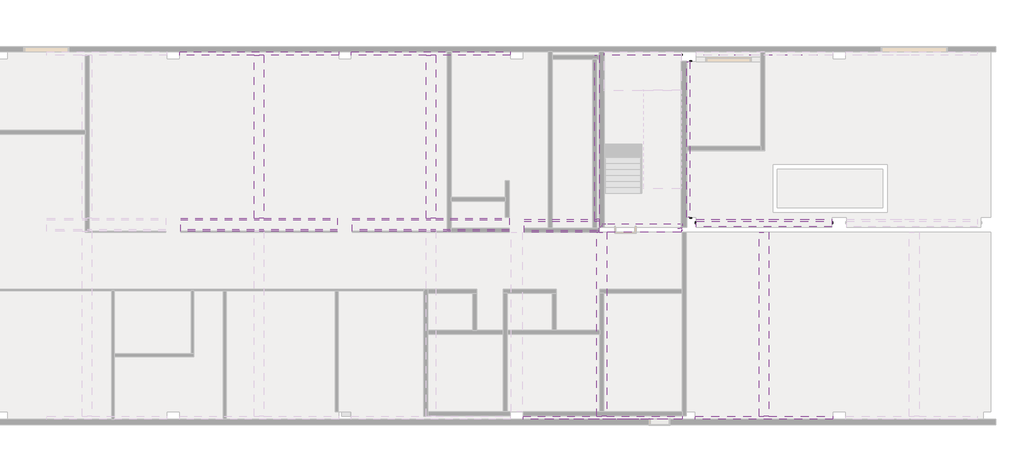
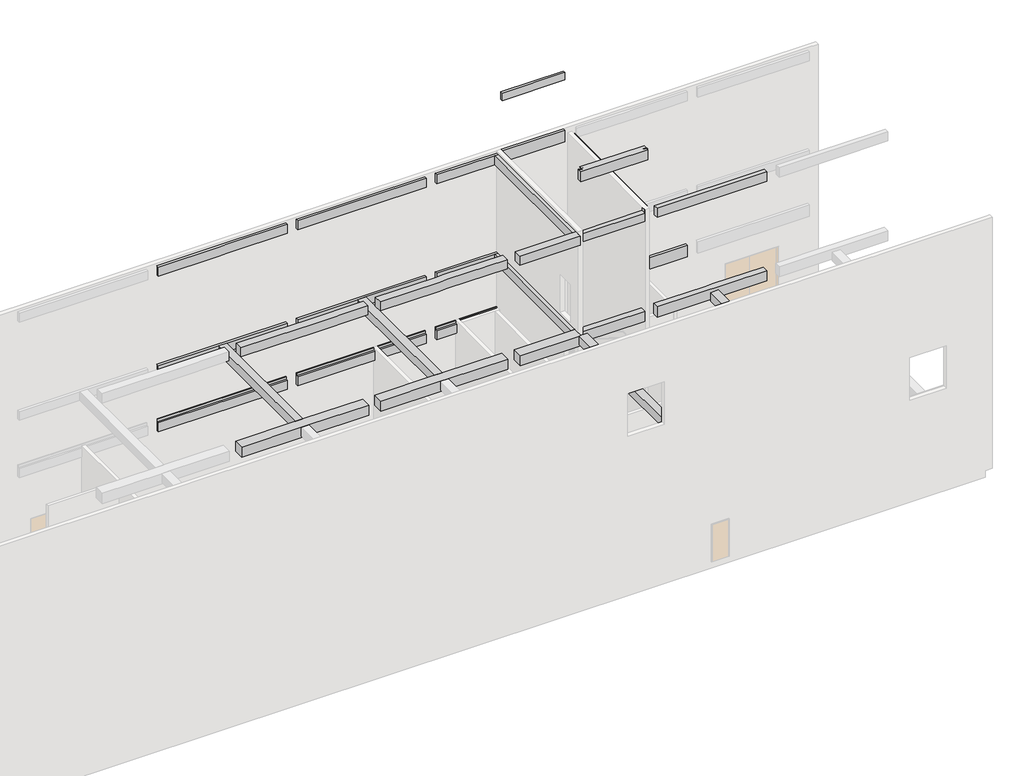
# One storey, part 4 of 5: 55 beams.
# Revit data of these elements (continued)
# Type "RC Beam_Rectangular : H_SB_AR_S16_UG_B500xH700_1G3" (continued)
#   H_WM Code_3 = "A03AF036-00001 |  | M2 | Concrete Work | Superstructure Work | Form Work (1 time in use) | Flat Form | Dressed Lumber, Plywood or Steel Form(Wood Planks are not Allowed) incl. Chamfer |  |  |  | A03AF036-00001 Concrete Work Superstructure Work Form Work (1 time in use) Flat Form     Dressed Lumber, Plywood or Steel Form(Wood Planks are not Allowed) incl. Chamfer   |"
#   중앙부 하부근 = ""
#   중앙부 상부근 = ""
#   중앙부 보조근 = ""
#   중앙부 늑근 = ""
#   외단부 하부근 = ""
#   외단부 상부근 = ""
#   외단부 보조근 = ""
#   외단부 늑근 = ""
#   부호 = "TG2"
#   내단부 하부근 = ""
#   내단부 상부근 = ""
#   내단부 보조근 = ""
#   내단부 늑근 = ""
#   ALL 하부근 = "3-D20"
#   ALL 상부근 = "4-D20"
#   ALL 보조근 = ""
#   ALL 늑근 = "2-D10 @120"
#   H_Rebar ratio = 0.14
#   Width = 500 mm
#   Height = 700 mm
#   Length [instance default] = 1524 mm
#   b = 500 mm
#   h = 700 mm
#   hec_material3 [instance default] = none
#   hec_material2 [instance default] = none
#   hec_material1 [instance default] = none
#   Structural Material [instance default] = none
#   Assembly Code = ""
# Type "RC Beam_Rectangular : H_SB_AR_S16_UG_B600xH800_1G2"
#   Type Comments = "CV-UG"
#   Type Mark = "1G2"
#   H_Q'ty Cal Type Tag = "SB-Q1"
#   H_WM Code_1 = "A03AF032-00022 |  | M3 | Concrete Work | Superstructure Work | Structural Concrete | Cement Type-1 | 25MPa ≤ F'c (Cylinder Strength) < 30MPa |  |  |  |  | A03AF032-00022 Concrete Work Superstructure Work Structural Concrete  Cement Type-1 25MPa ≤ F'c (Cylinder Strength) < 30MPa      |  F'c (Cylinder Strength) = 24MPa"
#   H_WM Code_2 = "A03AD037-00002 |  | TON | Concrete Work | Substructure Work | Rebar Work | Deformed Bar (Non-Coat.) | 400MPa<Fy≤470MPa |  |  |  |  | A03AD037-00002 Concrete Work Substructure Work Rebar Work Deformed Bar (Non-Coat.)  400MPa<Fy≤470MPa      | ASTM A615 GRADE 60 (Fy=420MPa)"
#   H_WM Code_3 = "A03AF036-00001 |  | M2 | Concrete Work | Superstructure Work | Form Work (1 time in use) | Flat Form | Dressed Lumber, Plywood or Steel Form(Wood Planks are not Allowed) incl. Chamfer |  |  |  | A03AF036-00001 Concrete Work Superstructure Work Form Work (1 time in use) Flat Form     Dressed Lumber, Plywood or Steel Form(Wood Planks are not Allowed) incl. Chamfer   |"
#   중앙부 하부근 = ""
#   중앙부 상부근 = ""
#   중앙부 보조근 = ""
#   중앙부 늑근 = ""
#   외단부 하부근 = ""
#   외단부 상부근 = ""
#   외단부 보조근 = ""
#   외단부 늑근 = ""
#   부호 = "TG2"
#   내단부 하부근 = ""
#   내단부 상부근 = ""
#   내단부 보조근 = ""
#   내단부 늑근 = ""
#   ALL 하부근 = "3-D20"
#   ALL 상부근 = "4-D20"
#   ALL 보조근 = ""
#   ALL 늑근 = "2-D10 @120"
#   H_Rebar ratio = 0.14
#   Width = 600 mm
#   Height = 800 mm
#   Length [instance default] = 1524 mm
#   b = 600 mm
#   h = 800 mm
#   hec_material3 [instance default] = none
#   hec_material2 [instance default] = none
#   hec_material1 [instance default] = none
#   Structural Material [instance default] = none
#   Assembly Code = ""
# Type "RC Beam_Rectangular : H_SB_AR_S16_UG_B450xH700_1B1"
#   Type Comments = "CV-UG"
#   Type Mark = "1B1"
#   H_Q'ty Cal Type Tag = "SB-Q1"
#   H_WM Code_1 = "A03AF032-00022 |  | M3 | Concrete Work | Superstructure Work | Structural Concrete | Cement Type-1 | 25MPa ≤ F'c (Cylinder Strength) < 30MPa |  |  |  |  | A03AF032-00022 Concrete Work Superstructure Work Structural Concrete  Cement Type-1 25MPa ≤ F'c (Cylinder Strength) < 30MPa      |  F'c (Cylinder Strength) = 24MPa"
#   H_WM Code_2 = "A03AD037-00002 |  | TON | Concrete Work | Substructure Work | Rebar Work | Deformed Bar (Non-Coat.) | 400MPa<Fy≤470MPa |  |  |  |  | A03AD037-00002 Concrete Work Substructure Work Rebar Work Deformed Bar (Non-Coat.)  400MPa<Fy≤470MPa      | ASTM A615 GRADE 60 (Fy=420MPa)"
#   H_WM Code_3 = "A03AF036-00001 |  | M2 | Concrete Work | Superstructure Work | Form Work (1 time in use) | Flat Form | Dressed Lumber, Plywood or Steel Form(Wood Planks are not Allowed) incl. Chamfer |  |  |  | A03AF036-00001 Concrete Work Superstructure Work Form Work (1 time in use) Flat Form     Dressed Lumber, Plywood or Steel Form(Wood Planks are not Allowed) incl. Chamfer   |"
#   중앙부 하부근 = ""
#   중앙부 상부근 = ""
#   중앙부 보조근 = ""
#   중앙부 늑근 = ""
#   외단부 하부근 = ""
#   외단부 상부근 = ""
#   외단부 보조근 = ""
#   외단부 늑근 = ""
#   부호 = "TG2"
#   내단부 하부근 = ""
#   내단부 상부근 = ""
#   내단부 보조근 = ""
#   내단부 늑근 = ""
#   ALL 하부근 = "3-D20"
#   ALL 상부근 = "4-D20"
#   ALL 보조근 = ""
#   ALL 늑근 = "2-D10 @120"
#   H_Rebar ratio = 0.14
#   Width = 450 mm
#   Height = 700 mm
#   Length [instance default] = 1524 mm
#   b = 450 mm
#   h = 700 mm
#   hec_material3 [instance default] = none
#   hec_material2 [instance default] = none
#   hec_material1 [instance default] = none
#   Structural Material [instance default] = none
#   Assembly Code = ""
# Type "RC Beam_Rectangular : H_SB_AR_S16_AG_B400xH700_3WG1"
#   Type Comments = "CV-AG"
#   Type Mark = "3WG1"
#   H_Q'ty Cal Type Tag = "SB-Q1"
#   H_WM Code_1 = "A03AF032-00022 |  | M3 | Concrete Work | Superstructure Work | Structural Concrete | Cement Type-1 | 25MPa ≤ F'c (Cylinder Strength) < 30MPa |  |  |  |  | A03AF032-00022 Concrete Work Superstructure Work Structural Concrete  Cement Type-1 25MPa ≤ F'c (Cylinder Strength) < 30MPa      |  F'c (Cylinder Strength) = 24MPa"
#   H_WM Code_2 = "A03AD037-00002 |  | TON | Concrete Work | Substructure Work | Rebar Work | Deformed Bar (Non-Coat.) | 400MPa<Fy≤470MPa |  |  |  |  | A03AD037-00002 Concrete Work Substructure Work Rebar Work Deformed Bar (Non-Coat.)  400MPa<Fy≤470MPa      | ASTM A615 GRADE 60 (Fy=420MPa)"
#   H_WM Code_3 = "A03AF036-00001 |  | M2 | Concrete Work | Superstructure Work | Form Work (1 time in use) | Flat Form | Dressed Lumber, Plywood or Steel Form(Wood Planks are not Allowed) incl. Chamfer |  |  |  | A03AF036-00001 Concrete Work Superstructure Work Form Work (1 time in use) Flat Form     Dressed Lumber, Plywood or Steel Form(Wood Planks are not Allowed) incl. Chamfer   |"
#   중앙부 하부근 = ""
#   중앙부 상부근 = ""
#   중앙부 보조근 = ""
#   중앙부 늑근 = ""
#   외단부 하부근 = ""
#   외단부 상부근 = ""
#   외단부 보조근 = ""
#   외단부 늑근 = ""
#   부호 = "TG2"
#   내단부 하부근 = ""
#   내단부 상부근 = ""
#   내단부 보조근 = ""
#   내단부 늑근 = ""
#   ALL 하부근 = "3-D20"
#   ALL 상부근 = "4-D20"
#   ALL 보조근 = ""
#   ALL 늑근 = "2-D10 @120"
#   H_Rebar ratio = 0.14
#   Width = 400 mm
#   Height = 700 mm
#   Length [instance default] = 1524 mm
#   b = 400 mm
#   h = 700 mm
#   hec_material3 [instance default] = none
#   hec_material2 [instance default] = none
#   hec_material1 [instance default] = none
#   Structural Material [instance default] = none
#   Assembly Code = ""
# Type "RC Beam_Rectangular : H_SB_AR_S16_AG_B600xH800_3G2"
#   Type Comments = "AG"
#   Type Mark = "3G2"
#   H_Q'ty Cal Type Tag = "SB-Q1"
#   H_WM Code_1 = "A03AF032-00022 |  | M3 | Concrete Work | Superstructure Work | Structural Concrete | Cement Type-1 | 25MPa ≤ F'c (Cylinder Strength) < 30MPa |  |  |  |  | A03AF032-00022 Concrete Work Superstructure Work Structural Concrete  Cement Type-1 25MPa ≤ F'c (Cylinder Strength) < 30MPa      |  F'c (Cylinder Strength) = 24MPa"
#   H_WM Code_2 = "A03AD037-00002 |  | TON | Concrete Work | Substructure Work | Rebar Work | Deformed Bar (Non-Coat.) | 400MPa<Fy≤470MPa |  |  |  |  | A03AD037-00002 Concrete Work Substructure Work Rebar Work Deformed Bar (Non-Coat.)  400MPa<Fy≤470MPa      | ASTM A615 GRADE 60 (Fy=420MPa)"
#   H_WM Code_3 = "A03AF036-00001 |  | M2 | Concrete Work | Superstructure Work | Form Work (1 time in use) | Flat Form | Dressed Lumber, Plywood or Steel Form(Wood Planks are not Allowed) incl. Chamfer |  |  |  | A03AF036-00001 Concrete Work Superstructure Work Form Work (1 time in use) Flat Form     Dressed Lumber, Plywood or Steel Form(Wood Planks are not Allowed) incl. Chamfer   |"
#   중앙부 하부근 = ""
#   중앙부 상부근 = ""
#   중앙부 보조근 = ""
#   중앙부 늑근 = ""
#   외단부 하부근 = ""
#   외단부 상부근 = ""
#   외단부 보조근 = ""
#   외단부 늑근 = ""
#   부호 = "TG2"
#   내단부 하부근 = ""
#   내단부 상부근 = ""
#   내단부 보조근 = ""
#   내단부 늑근 = ""
#   ALL 하부근 = "3-D20"
#   ALL 상부근 = "4-D20"
#   ALL 보조근 = ""
#   ALL 늑근 = "2-D10 @120"
#   Width = 600 mm
#   Height = 800 mm
#   Length [instance default] = 1524 mm
#   b = 600 mm
#   h = 800 mm
#   hec_material3 [instance default] = none
#   hec_material2 [instance default] = none
#   hec_material1 [instance default] = none
#   Structural Material [instance default] = none
#   Assembly Code = ""
# Type "RC Beam_Rectangular : H_SB_AR_S16_AG_B600xH800_3WG2"
#   Type Comments = "AG"
#   Type Mark = "3WG2"
#   H_Q'ty Cal Type Tag = "SB-Q1"
#   H_WM Code_1 = "A03AF032-00022 |  | M3 | Concrete Work | Superstructure Work | Structural Concrete | Cement Type-1 | 25MPa ≤ F'c (Cylinder Strength) < 30MPa |  |  |  |  | A03AF032-00022 Concrete Work Superstructure Work Structural Concrete  Cement Type-1 25MPa ≤ F'c (Cylinder Strength) < 30MPa      |  F'c (Cylinder Strength) = 24MPa"
#   H_WM Code_2 = "A03AD037-00002 |  | TON | Concrete Work | Substructure Work | Rebar Work | Deformed Bar (Non-Coat.) | 400MPa<Fy≤470MPa |  |  |  |  | A03AD037-00002 Concrete Work Substructure Work Rebar Work Deformed Bar (Non-Coat.)  400MPa<Fy≤470MPa      | ASTM A615 GRADE 60 (Fy=420MPa)"
#   H_WM Code_3 = "A03AF036-00001 |  | M2 | Concrete Work | Superstructure Work | Form Work (1 time in use) | Flat Form | Dressed Lumber, Plywood or Steel Form(Wood Planks are not Allowed) incl. Chamfer |  |  |  | A03AF036-00001 Concrete Work Superstructure Work Form Work (1 time in use) Flat Form     Dressed Lumber, Plywood or Steel Form(Wood Planks are not Allowed) incl. Chamfer   |"
#   중앙부 하부근 = ""
#   중앙부 상부근 = ""
#   중앙부 보조근 = ""
#   중앙부 늑근 = ""
#   외단부 하부근 = ""
#   외단부 상부근 = ""
#   외단부 보조근 = ""
#   외단부 늑근 = ""
#   부호 = "TG2"
#   내단부 하부근 = ""
#   내단부 상부근 = ""
#   내단부 보조근 = ""
#   내단부 늑근 = ""
#   ALL 하부근 = "3-D20"
#   ALL 상부근 = "4-D20"
#   ALL 보조근 = ""
#   ALL 늑근 = "2-D10 @120"
#   Width = 600 mm
#   Height = 800 mm
#   Length [instance default] = 1524 mm
#   b = 600 mm
#   h = 800 mm
#   hec_material3 [instance default] = none
#   hec_material2 [instance default] = none
#   hec_material1 [instance default] = none
#   Structural Material [instance default] = none
#   Assembly Code = ""
# Type "RC Beam_Rectangular : H_SB_AR_S16_AG_B400xH700_3WG3"
#   Type Comments = "AG"
#   Type Mark = "3WG3"
#   H_Q'ty Cal Type Tag = "SB-Q1"
#   H_WM Code_1 = "A03AF032-00022 |  | M3 | Concrete Work | Superstructure Work | Structural Concrete | Cement Type-1 | 25MPa ≤ F'c (Cylinder Strength) < 30MPa |  |  |  |  | A03AF032-00022 Concrete Work Superstructure Work Structural Concrete  Cement Type-1 25MPa ≤ F'c (Cylinder Strength) < 30MPa      |  F'c (Cylinder Strength) = 24MPa"
#   H_WM Code_2 = "A03AD037-00002 |  | TON | Concrete Work | Substructure Work | Rebar Work | Deformed Bar (Non-Coat.) | 400MPa<Fy≤470MPa |  |  |  |  | A03AD037-00002 Concrete Work Substructure Work Rebar Work Deformed Bar (Non-Coat.)  400MPa<Fy≤470MPa      | ASTM A615 GRADE 60 (Fy=420MPa)"
#   H_WM Code_3 = "A03AF036-00001 |  | M2 | Concrete Work | Superstructure Work | Form Work (1 time in use) | Flat Form | Dressed Lumber, Plywood or Steel Form(Wood Planks are not Allowed) incl. Chamfer |  |  |  | A03AF036-00001 Concrete Work Superstructure Work Form Work (1 time in use) Flat Form     Dressed Lumber, Plywood or Steel Form(Wood Planks are not Allowed) incl. Chamfer   |"
#   중앙부 하부근 = ""
#   중앙부 상부근 = ""
#   중앙부 보조근 = ""
#   중앙부 늑근 = ""
#   외단부 하부근 = ""
#   외단부 상부근 = ""
#   외단부 보조근 = ""
#   외단부 늑근 = ""
#   부호 = "TG2"
#   내단부 하부근 = ""
#   내단부 상부근 = ""
#   내단부 보조근 = ""
#   내단부 늑근 = ""
#   ALL 하부근 = "3-D20"
#   ALL 상부근 = "4-D20"
#   ALL 보조근 = ""
#   ALL 늑근 = "2-D10 @120"
#   Width = 400 mm
#   Height = 700 mm
#   Length [instance default] = 1524 mm
#   b = 400 mm
#   h = 700 mm
#   hec_material3 [instance default] = none
#   hec_material2 [instance default] = none
#   hec_material1 [instance default] = none
#   Structural Material [instance default] = none
#   Assembly Code = ""
# Type "RC Beam_Rectangular : H_SB_AR_S16_AG_B450xH700_2WB1"
#   Type Comments = "AG"
#   Type Mark = "2WB1"
#   H_Q'ty Cal Type Tag = "SB-Q1"
#   H_WM Code_1 = "A03AF032-00022 |  | M3 | Concrete Work | Superstructure Work | Structural Concrete | Cement Type-1 | 25MPa ≤ F'c (Cylinder Strength) < 30MPa |  |  |  |  | A03AF032-00022 Concrete Work Superstructure Work Structural Concrete  Cement Type-1 25MPa ≤ F'c (Cylinder Strength) < 30MPa      |  F'c (Cylinder Strength) = 24MPa"
#   H_WM Code_2 = "A03AD037-00002 |  | TON | Concrete Work | Substructure Work | Rebar Work | Deformed Bar (Non-Coat.) | 400MPa<Fy≤470MPa |  |  |  |  | A03AD037-00002 Concrete Work Substructure Work Rebar Work Deformed Bar (Non-Coat.)  400MPa<Fy≤470MPa      | ASTM A615 GRADE 60 (Fy=420MPa)"
#   H_WM Code_3 = "A03AF036-00001 |  | M2 | Concrete Work | Superstructure Work | Form Work (1 time in use) | Flat Form | Dressed Lumber, Plywood or Steel Form(Wood Planks are not Allowed) incl. Chamfer |  |  |  | A03AF036-00001 Concrete Work Superstructure Work Form Work (1 time in use) Flat Form     Dressed Lumber, Plywood or Steel Form(Wood Planks are not Allowed) incl. Chamfer   |"
#   중앙부 하부근 = ""
#   중앙부 상부근 = ""
#   중앙부 보조근 = ""
#   중앙부 늑근 = ""
#   외단부 하부근 = ""
#   외단부 상부근 = ""
#   외단부 보조근 = ""
#   외단부 늑근 = ""
#   부호 = "TG2"
#   내단부 하부근 = ""
#   내단부 상부근 = ""
#   내단부 보조근 = ""
#   내단부 늑근 = ""
#   ALL 하부근 = "3-D20"
#   ALL 상부근 = "4-D20"
#   ALL 보조근 = ""
#   ALL 늑근 = "2-D10 @120"
#   Width = 450 mm
#   Height = 700 mm
#   Length [instance default] = 1524 mm
#   b = 450 mm
#   h = 700 mm
#   hec_material3 [instance default] = none
#   hec_material2 [instance default] = none
#   hec_material1 [instance default] = none
#   Structural Material [instance default] = none
#   Assembly Code = ""
# Type "RC Beam_Rectangular : H_SB_AR_S16_AG_B450xH700_3B1"
#   Type Comments = "AG"
#   Type Mark = "3B1"
#   H_Q'ty Cal Type Tag = "SB-Q1"
#   H_WM Code_1 = "A03AF032-00022 |  | M3 | Concrete Work | Superstructure Work | Structural Concrete | Cement Type-1 | 25MPa ≤ F'c (Cylinder Strength) < 30MPa |  |  |  |  | A03AF032-00022 Concrete Work Superstructure Work Structural Concrete  Cement Type-1 25MPa ≤ F'c (Cylinder Strength) < 30MPa      |  F'c (Cylinder Strength) = 24MPa"
#   H_WM Code_2 = "A03AD037-00002 |  | TON | Concrete Work | Substructure Work | Rebar Work | Deformed Bar (Non-Coat.) | 400MPa<Fy≤470MPa |  |  |  |  | A03AD037-00002 Concrete Work Substructure Work Rebar Work Deformed Bar (Non-Coat.)  400MPa<Fy≤470MPa      | ASTM A615 GRADE 60 (Fy=420MPa)"
#   H_WM Code_3 = "A03AF036-00001 |  | M2 | Concrete Work | Superstructure Work | Form Work (1 time in use) | Flat Form | Dressed Lumber, Plywood or Steel Form(Wood Planks are not Allowed) incl. Chamfer |  |  |  | A03AF036-00001 Concrete Work Superstructure Work Form Work (1 time in use) Flat Form     Dressed Lumber, Plywood or Steel Form(Wood Planks are not Allowed) incl. Chamfer   |"
#   중앙부 하부근 = ""
#   중앙부 상부근 = ""
#   중앙부 보조근 = ""
#   중앙부 늑근 = ""
#   외단부 하부근 = ""
#   외단부 상부근 = ""
#   외단부 보조근 = ""
#   외단부 늑근 = ""
#   부호 = "TG2"
#   내단부 하부근 = ""
#   내단부 상부근 = ""
#   내단부 보조근 = ""
#   내단부 늑근 = ""
#   ALL 하부근 = "3-D20"
#   ALL 상부근 = "4-D20"
#   ALL 보조근 = ""
#   ALL 늑근 = "2-D10 @120"
#   Width = 450 mm
#   Height = 700 mm
#   Length [instance default] = 1524 mm
#   b = 450 mm
#   h = 700 mm
#   hec_material3 [instance default] = none
#   hec_material2 [instance default] = none
#   hec_material1 [instance default] = none
#   Structural Material [instance default] = none
#   Assembly Code = ""
# Type "RC Beam_Rectangular : H_SB_AR_S16_AG_B450xH700_3WB1"
#   Type Comments = "AG"
#   Type Mark = "3WB1"
#   H_Q'ty Cal Type Tag = "SB-Q1"
#   H_WM Code_1 = "A03AF032-00022 |  | M3 | Concrete Work | Superstructure Work | Structural Concrete | Cement Type-1 | 25MPa ≤ F'c (Cylinder Strength) < 30MPa |  |  |  |  | A03AF032-00022 Concrete Work Superstructure Work Structural Concrete  Cement Type-1 25MPa ≤ F'c (Cylinder Strength) < 30MPa      |  F'c (Cylinder Strength) = 24MPa"
#   H_WM Code_2 = "A03AD037-00002 |  | TON | Concrete Work | Substructure Work | Rebar Work | Deformed Bar (Non-Coat.) | 400MPa<Fy≤470MPa |  |  |  |  | A03AD037-00002 Concrete Work Substructure Work Rebar Work Deformed Bar (Non-Coat.)  400MPa<Fy≤470MPa      | ASTM A615 GRADE 60 (Fy=420MPa)"
#   H_WM Code_3 = "A03AF036-00001 |  | M2 | Concrete Work | Superstructure Work | Form Work (1 time in use) | Flat Form | Dressed Lumber, Plywood or Steel Form(Wood Planks are not Allowed) incl. Chamfer |  |  |  | A03AF036-00001 Concrete Work Superstructure Work Form Work (1 time in use) Flat Form     Dressed Lumber, Plywood or Steel Form(Wood Planks are not Allowed) incl. Chamfer   |"
#   중앙부 하부근 = ""
#   중앙부 상부근 = ""
#   중앙부 보조근 = ""
#   중앙부 늑근 = ""
#   외단부 하부근 = ""
#   외단부 상부근 = ""
#   외단부 보조근 = ""
#   외단부 늑근 = ""
#   부호 = "TG2"
#   내단부 하부근 = ""
#   내단부 상부근 = ""
#   내단부 보조근 = ""
#   내단부 늑근 = ""
#   ALL 하부근 = "3-D20"
#   ALL 상부근 = "4-D20"
#   ALL 보조근 = ""
#   ALL 늑근 = "2-D10 @120"
#   Width = 450 mm
#   Height = 700 mm
#   Length [instance default] = 1524 mm
#   b = 450 mm
#   h = 700 mm
#   hec_material3 [instance default] = none
#   hec_material2 [instance default] = none
#   hec_material1 [instance default] = none
#   Structural Material [instance default] = none
#   Assembly Code = ""
# Type "RC Beam_Rectangular : H_SB_AR_S16_AG_B450xH700_3B1A"
#   Type Comments = "AG"
#   Type Mark = "3B1A"
#   H_Q'ty Cal Type Tag = "SB-Q1"
#   H_WM Code_1 = "A03AF032-00022 |  | M3 | Concrete Work | Superstructure Work | Structural Concrete | Cement Type-1 | 25MPa ≤ F'c (Cylinder Strength) < 30MPa |  |  |  |  | A03AF032-00022 Concrete Work Superstructure Work Structural Concrete  Cement Type-1 25MPa ≤ F'c (Cylinder Strength) < 30MPa      |  F'c (Cylinder Strength) = 24MPa"
#   H_WM Code_2 = "A03AD037-00002 |  | TON | Concrete Work | Substructure Work | Rebar Work | Deformed Bar (Non-Coat.) | 400MPa<Fy≤470MPa |  |  |  |  | A03AD037-00002 Concrete Work Substructure Work Rebar Work Deformed Bar (Non-Coat.)  400MPa<Fy≤470MPa      | ASTM A615 GRADE 60 (Fy=420MPa)"
#   H_WM Code_3 = "A03AF036-00001 |  | M2 | Concrete Work | Superstructure Work | Form Work (1 time in use) | Flat Form | Dressed Lumber, Plywood or Steel Form(Wood Planks are not Allowed) incl. Chamfer |  |  |  | A03AF036-00001 Concrete Work Superstructure Work Form Work (1 time in use) Flat Form     Dressed Lumber, Plywood or Steel Form(Wood Planks are not Allowed) incl. Chamfer   |"
#   중앙부 하부근 = ""
#   중앙부 상부근 = ""
#   중앙부 보조근 = ""
#   중앙부 늑근 = ""
#   외단부 하부근 = ""
#   외단부 상부근 = ""
#   외단부 보조근 = ""
#   외단부 늑근 = ""
#   부호 = "TG2"
#   내단부 하부근 = ""
#   내단부 상부근 = ""
#   내단부 보조근 = ""
#   내단부 늑근 = ""
#   ALL 하부근 = "3-D20"
#   ALL 상부근 = "4-D20"
#   ALL 보조근 = ""
#   ALL 늑근 = "2-D10 @120"
#   Width = 450 mm
#   Height = 700 mm
#   Length [instance default] = 1524 mm
#   b = 450 mm
#   h = 700 mm
#   hec_material3 [instance default] = none
#   hec_material2 [instance default] = none
#   hec_material1 [instance default] = none
#   Structural Material [instance default] = none
#   Assembly Code = ""
# Type "RC Beam_Rectangular : H_SB_AR_S16_AG_B400xH700_RWG1"
#   Type Comments = "CV-AG"
#   Type Mark = "RWG1"
#   H_Q'ty Cal Type Tag = "SB-Q1"
#   H_WM Code_1 = "A03AF032-00022 |  | M3 | Concrete Work | Superstructure Work | Structural Concrete | Cement Type-1 | 25MPa ≤ F'c (Cylinder Strength) < 30MPa |  |  |  |  | A03AF032-00022 Concrete Work Superstructure Work Structural Concrete  Cement Type-1 25MPa ≤ F'c (Cylinder Strength) < 30MPa      |  F'c (Cylinder Strength) = 24MPa"
#   H_WM Code_2 = "A03AD037-00002 |  | TON | Concrete Work | Substructure Work | Rebar Work | Deformed Bar (Non-Coat.) | 400MPa<Fy≤470MPa |  |  |  |  | A03AD037-00002 Concrete Work Substructure Work Rebar Work Deformed Bar (Non-Coat.)  400MPa<Fy≤470MPa      | ASTM A615 GRADE 60 (Fy=420MPa)"
#   H_WM Code_3 = "A03AF036-00001 |  | M2 | Concrete Work | Superstructure Work | Form Work (1 time in use) | Flat Form | Dressed Lumber, Plywood or Steel Form(Wood Planks are not Allowed) incl. Chamfer |  |  |  | A03AF036-00001 Concrete Work Superstructure Work Form Work (1 time in use) Flat Form     Dressed Lumber, Plywood or Steel Form(Wood Planks are not Allowed) incl. Chamfer   |"
#   중앙부 하부근 = ""
#   중앙부 상부근 = ""
#   중앙부 보조근 = ""
#   중앙부 늑근 = ""
#   외단부 하부근 = ""
#   외단부 상부근 = ""
#   외단부 보조근 = ""
#   외단부 늑근 = ""
#   부호 = "TG2"
#   내단부 하부근 = ""
#   내단부 상부근 = ""
#   내단부 보조근 = ""
#   내단부 늑근 = ""
#   ALL 하부근 = "3-D20"
#   ALL 상부근 = "4-D20"
#   ALL 보조근 = ""
#   ALL 늑근 = "2-D10 @120"
#   H_Rebar ratio = 0.14
#   Width = 400 mm
#   Height = 700 mm
#   Length [instance default] = 1524 mm
#   b = 400 mm
#   h = 700 mm
#   hec_material3 [instance default] = none
#   hec_material2 [instance default] = none
#   hec_material1 [instance default] = none
#   Structural Material [instance default] = none
#   Assembly Code = ""
# Type "RC Beam_Rectangular : H_SB_AR_S16_AG_B450xH700_RWG3"
#   Type Comments = "AG"
#   Type Mark = "RWG3"
#   H_Q'ty Cal Type Tag = "SB-Q1"
#   H_WM Code_1 = "A03AF032-00022 |  | M3 | Concrete Work | Superstructure Work | Structural Concrete | Cement Type-1 | 25MPa ≤ F'c (Cylinder Strength) < 30MPa |  |  |  |  | A03AF032-00022 Concrete Work Superstructure Work Structural Concrete  Cement Type-1 25MPa ≤ F'c (Cylinder Strength) < 30MPa      |  F'c (Cylinder Strength) = 24MPa"
#   H_WM Code_2 = "A03AD037-00002 |  | TON | Concrete Work | Substructure Work | Rebar Work | Deformed Bar (Non-Coat.) | 400MPa<Fy≤470MPa |  |  |  |  | A03AD037-00002 Concrete Work Substructure Work Rebar Work Deformed Bar (Non-Coat.)  400MPa<Fy≤470MPa      | ASTM A615 GRADE 60 (Fy=420MPa)"
#   H_WM Code_3 = "A03AF036-00001 |  | M2 | Concrete Work | Superstructure Work | Form Work (1 time in use) | Flat Form | Dressed Lumber, Plywood or Steel Form(Wood Planks are not Allowed) incl. Chamfer |  |  |  | A03AF036-00001 Concrete Work Superstructure Work Form Work (1 time in use) Flat Form     Dressed Lumber, Plywood or Steel Form(Wood Planks are not Allowed) incl. Chamfer   |"
#   중앙부 하부근 = ""
#   중앙부 상부근 = ""
#   중앙부 보조근 = ""
#   중앙부 늑근 = ""
#   외단부 하부근 = ""
#   외단부 상부근 = ""
#   외단부 보조근 = ""
#   외단부 늑근 = ""
#   부호 = "TG2"
#   내단부 하부근 = ""
#   내단부 상부근 = ""
#   내단부 보조근 = ""
#   내단부 늑근 = ""
#   ALL 하부근 = "3-D20"
#   ALL 상부근 = "4-D20"
#   ALL 보조근 = ""
#   ALL 늑근 = "2-D10 @120"
#   Width = 450 mm
#   Height = 700 mm
#   Length [instance default] = 1524 mm
#   b = 450 mm
#   h = 700 mm
#   hec_material3 [instance default] = none
#   hec_material2 [instance default] = none
#   hec_material1 [instance default] = none
#   Structural Material [instance default] = none
#   Assembly Code = ""
# Type "RC Beam_Rectangular : H_SB_AR_S16_AG_B400xH700_RWG4"
#   Type Comments = "AG"
#   Type Mark = "RWG4"
#   H_Q'ty Cal Type Tag = "SB-Q1"
#   H_WM Code_1 = "A03AF032-00022 |  | M3 | Concrete Work | Superstructure Work | Structural Concrete | Cement Type-1 | 25MPa ≤ F'c (Cylinder Strength) < 30MPa |  |  |  |  | A03AF032-00022 Concrete Work Superstructure Work Structural Concrete  Cement Type-1 25MPa ≤ F'c (Cylinder Strength) < 30MPa      |  F'c (Cylinder Strength) = 24MPa"
#   H_WM Code_2 = "A03AD037-00002 |  | TON | Concrete Work | Substructure Work | Rebar Work | Deformed Bar (Non-Coat.) | 400MPa<Fy≤470MPa |  |  |  |  | A03AD037-00002 Concrete Work Substructure Work Rebar Work Deformed Bar (Non-Coat.)  400MPa<Fy≤470MPa      | ASTM A615 GRADE 60 (Fy=420MPa)"
#   H_WM Code_3 = "A03AF036-00001 |  | M2 | Concrete Work | Superstructure Work | Form Work (1 time in use) | Flat Form | Dressed Lumber, Plywood or Steel Form(Wood Planks are not Allowed) incl. Chamfer |  |  |  | A03AF036-00001 Concrete Work Superstructure Work Form Work (1 time in use) Flat Form     Dressed Lumber, Plywood or Steel Form(Wood Planks are not Allowed) incl. Chamfer   |"
#   중앙부 하부근 = ""
#   중앙부 상부근 = ""
#   중앙부 보조근 = ""
#   중앙부 늑근 = ""
#   외단부 하부근 = ""
#   외단부 상부근 = ""
#   외단부 보조근 = ""
#   외단부 늑근 = ""
#   부호 = "TG2"
#   내단부 하부근 = ""
#   내단부 상부근 = ""
#   내단부 보조근 = ""
#   내단부 늑근 = ""
#   ALL 하부근 = "3-D20"
#   ALL 상부근 = "4-D20"
#   ALL 보조근 = ""
#   ALL 늑근 = "2-D10 @120"
#   Width = 400 mm
#   Height = 700 mm
#   Length [instance default] = 1524 mm
#   b = 400 mm
#   h = 700 mm
#   hec_material3 [instance default] = none
#   hec_material2 [instance default] = none
#   hec_material1 [instance default] = none
#   Structural Material [instance default] = none
#   Assembly Code = ""
# Type "RC Beam_Rectangular : H_SB_AR_S16_AG_B450xH700_RWB1"
#   Type Comments = "AG"
#   Type Mark = "RWB1"
#   H_Q'ty Cal Type Tag = "SB-Q1"
#   H_WM Code_1 = "A03AF032-00022 |  | M3 | Concrete Work | Superstructure Work | Structural Concrete | Cement Type-1 | 25MPa ≤ F'c (Cylinder Strength) < 30MPa |  |  |  |  | A03AF032-00022 Concrete Work Superstructure Work Structural Concrete  Cement Type-1 25MPa ≤ F'c (Cylinder Strength) < 30MPa      |  F'c (Cylinder Strength) = 24MPa"
#   H_WM Code_2 = "A03AD037-00002 |  | TON | Concrete Work | Substructure Work | Rebar Work | Deformed Bar (Non-Coat.) | 400MPa<Fy≤470MPa |  |  |  |  | A03AD037-00002 Concrete Work Substructure Work Rebar Work Deformed Bar (Non-Coat.)  400MPa<Fy≤470MPa      | ASTM A615 GRADE 60 (Fy=420MPa)"
#   H_WM Code_3 = "A03AF036-00001 |  | M2 | Concrete Work | Superstructure Work | Form Work (1 time in use) | Flat Form | Dressed Lumber, Plywood or Steel Form(Wood Planks are not Allowed) incl. Chamfer |  |  |  | A03AF036-00001 Concrete Work Superstructure Work Form Work (1 time in use) Flat Form     Dressed Lumber, Plywood or Steel Form(Wood Planks are not Allowed) incl. Chamfer   |"
#   중앙부 하부근 = ""
#   중앙부 상부근 = ""
#   중앙부 보조근 = ""
#   중앙부 늑근 = ""
#   외단부 하부근 = ""
#   외단부 상부근 = ""
#   외단부 보조근 = ""
#   외단부 늑근 = ""
#   부호 = "TG2"
#   내단부 하부근 = ""
#   내단부 상부근 = ""
#   내단부 보조근 = ""
#   내단부 늑근 = ""
#   ALL 하부근 = "3-D20"
#   ALL 상부근 = "4-D20"
#   ALL 보조근 = ""
#   ALL 늑근 = "2-D10 @120"
#   Width = 450 mm
#   Height = 700 mm
#   Length [instance default] = 1524 mm
#   b = 450 mm
#   h = 700 mm
#   hec_material3 [instance default] = none
#   hec_material2 [instance default] = none
#   hec_material1 [instance default] = none
#   Structural Material [instance default] = none
#   Assembly Code = ""
# Type "RC Beam_Rectangular : H_SB_AR_S16_AG_B450xH700_RG2"
#   Type Comments = "AG"
#   Type Mark = "RG2"
#   H_Q'ty Cal Type Tag = "SB-Q1"
#   H_WM Code_1 = "A03AF032-00022 |  | M3 | Concrete Work | Superstructure Work | Structural Concrete | Cement Type-1 | 25MPa ≤ F'c (Cylinder Strength) < 30MPa |  |  |  |  | A03AF032-00022 Concrete Work Superstructure Work Structural Concrete  Cement Type-1 25MPa ≤ F'c (Cylinder Strength) < 30MPa      |  F'c (Cylinder Strength) = 24MPa"
#   H_WM Code_2 = "A03AD037-00002 |  | TON | Concrete Work | Substructure Work | Rebar Work | Deformed Bar (Non-Coat.) | 400MPa<Fy≤470MPa |  |  |  |  | A03AD037-00002 Concrete Work Substructure Work Rebar Work Deformed Bar (Non-Coat.)  400MPa<Fy≤470MPa      | ASTM A615 GRADE 60 (Fy=420MPa)"
#   H_WM Code_3 = "A03AF036-00001 |  | M2 | Concrete Work | Superstructure Work | Form Work (1 time in use) | Flat Form | Dressed Lumber, Plywood or Steel Form(Wood Planks are not Allowed) incl. Chamfer |  |  |  | A03AF036-00001 Concrete Work Superstructure Work Form Work (1 time in use) Flat Form     Dressed Lumber, Plywood or Steel Form(Wood Planks are not Allowed) incl. Chamfer   |"
#   중앙부 하부근 = ""
#   중앙부 상부근 = ""
#   중앙부 보조근 = ""
#   중앙부 늑근 = ""
#   외단부 하부근 = ""
#   외단부 상부근 = ""
#   외단부 보조근 = ""
#   외단부 늑근 = ""
#   부호 = "TG2"
#   내단부 하부근 = ""
#   내단부 상부근 = ""
#   내단부 보조근 = ""
#   내단부 늑근 = ""
#   ALL 하부근 = "3-D20"
#   ALL 상부근 = "4-D20"
#   ALL 보조근 = ""
#   ALL 늑근 = "2-D10 @120"
#   Width = 450 mm
#   Height = 700 mm
#   Length [instance default] = 1524 mm
#   b = 450 mm
#   h = 700 mm
#   hec_material3 [instance default] = none
#   hec_material2 [instance default] = none
#   hec_material1 [instance default] = none
#   Structural Material [instance default] = none
#   Assembly Code = ""
# Type "RC Beam_Rectangular : H_SB_AR_S16_AG_B400xH600_PHWG2"
#   Type Comments = "CV-AG"
#   Type Mark = "PHWG2"
#   H_Q'ty Cal Type Tag = "SB-Q1"
#   H_WM Code_1 = "A03AF032-00022 |  | M3 | Concrete Work | Superstructure Work | Structural Concrete | Cement Type-1 | 25MPa ≤ F'c (Cylinder Strength) < 30MPa |  |  |  |  | A03AF032-00022 Concrete Work Superstructure Work Structural Concrete  Cement Type-1 25MPa ≤ F'c (Cylinder Strength) < 30MPa      |  F'c (Cylinder Strength) = 24MPa"
#   H_WM Code_2 = "A03AD037-00002 |  | TON | Concrete Work | Substructure Work | Rebar Work | Deformed Bar (Non-Coat.) | 400MPa<Fy≤470MPa |  |  |  |  | A03AD037-00002 Concrete Work Substructure Work Rebar Work Deformed Bar (Non-Coat.)  400MPa<Fy≤470MPa      | ASTM A615 GRADE 60 (Fy=420MPa)"
#   H_WM Code_3 = "A03AF036-00001 |  | M2 | Concrete Work | Superstructure Work | Form Work (1 time in use) | Flat Form | Dressed Lumber, Plywood or Steel Form(Wood Planks are not Allowed) incl. Chamfer |  |  |  | A03AF036-00001 Concrete Work Superstructure Work Form Work (1 time in use) Flat Form     Dressed Lumber, Plywood or Steel Form(Wood Planks are not Allowed) incl. Chamfer   |"
#   중앙부 하부근 = ""
#   중앙부 상부근 = ""
#   중앙부 보조근 = ""
#   중앙부 늑근 = ""
#   외단부 하부근 = ""
#   외단부 상부근 = ""
#   외단부 보조근 = ""
#   외단부 늑근 = ""
#   부호 = "TG2"
#   내단부 하부근 = ""
#   내단부 상부근 = ""
#   내단부 보조근 = ""
#   내단부 늑근 = ""
#   ALL 하부근 = "3-D20"
#   ALL 상부근 = "4-D20"
#   ALL 보조근 = ""
#   ALL 늑근 = "2-D10 @120"
#   H_Rebar ratio = 0.14
#   Width = 400 mm
#   Height = 600 mm
#   Length [instance default] = 1524 mm
#   b = 400 mm
#   h = 600 mm
#   hec_material3 [instance default] = none
#   hec_material2 [instance default] = none
#   hec_material1 [instance default] = none
#   Structural Material [instance default] = none
#   Assembly Code = ""
# Elements 1, 2, 12, 13 (IfcBeam, "RC Beam_Rectangular : H_SB_AR_S16_UG_B500xH700_1G1")
#   Comments = ""
#   hec_material3 = none
#   hec_material2 = none
#   hec_material1 = none
#   Structural Material = 00_Concrete_Reinf. Conc.
#   Phase Created = New Construction
#   Materials on its faces: "00_Concrete_Reinf. Conc."
# Elements 3, 4 (IfcBeam, "RC Beam_Rectangular : H_SB_AR_S16_UG_B450xH700_1B2")
#   Comments = ""
#   hec_material3 = none
#   hec_material2 = none
#   hec_material1 = none
#   Structural Material = 00_Concrete_Reinf. Conc.
#   Phase Created = New Construction
#   Materials on its faces: "00_Concrete_Reinf. Conc."
# Element 5 (IfcBeam, "RC Beam_Rectangular : H_SB_AR_S16_UG_B450xH700_1B1A")
#   Comments = ""
#   hec_material3 = none
#   hec_material2 = none
#   hec_material1 = none
#   Structural Material = none
#   Phase Created = New Construction
# Element 6 (IfcBeam, "RC Beam_Rectangular : H_SB_AR_S16_UG_B500xH700_1G3")
#   Comments = ""
#   hec_material3 = none
#   hec_material2 = none
#   hec_material1 = none
#   Structural Material = none
#   Phase Created = New Construction
# Elements 7, 8, 9 (IfcBeam, "RC Beam_Rectangular : H_SB_AR_S16_UG_B600xH800_1G2")
#   Comments = ""
#   hec_material3 = none
#   hec_material2 = none
#   hec_material1 = none
#   Structural Material = 00_Concrete_Reinf. Conc.
#   Phase Created = New Construction
#   Materials on its faces: "00_Concrete_Reinf. Conc."
# Elements 10, 11 (IfcBeam, "RC Beam_Rectangular : H_SB_AR_S16_UG_B450xH700_1B1")
#   Comments = ""
#   hec_material3 = none
#   hec_material2 = none
#   hec_material1 = none
#   Structural Material = 00_Concrete_Reinf. Conc.
#   Phase Created = New Construction
#   Materials on its faces: "00_Concrete_Reinf. Conc."
# Element 14 (IfcBeam, "RC Beam_Rectangular : H_SB_AR_S16_UG_B500xH700_1G1")
#   Comments = ""
#   hec_material3 = none
#   hec_material2 = none
#   hec_material1 = none
#   Structural Material = none
#   Phase Created = New Construction
# Elements 15, 16, 17, 18, 19, 20, 28, 29, 30, 31, 32 (IfcBeam, "RC Beam_Rectangular : H_SB_AR_S16_AG_B400xH700_3WG1")
#   Comments = ""
#   hec_material3 = none
#   hec_material2 = none
#   hec_material1 = none
#   Structural Material = 00_Concrete_Reinf. Conc.
#   Phase Created = New Construction
#   Materials on its faces: "00_Concrete_Reinf. Conc."
# Elements 21, 22, 33, 34 (IfcBeam, "RC Beam_Rectangular : H_SB_AR_S16_AG_B600xH800_3G2")
#   Comments = ""
#   hec_material3 = none
#   hec_material2 = none
#   hec_material1 = none
#   Structural Material = none
#   Phase Created = New Construction
# Elements 23, 24, 35, 36 (IfcBeam, "RC Beam_Rectangular : H_SB_AR_S16_AG_B600xH800_3WG2")
#   Comments = ""
#   hec_material3 = none
#   hec_material2 = none
#   hec_material1 = none
#   Structural Material = none
#   Phase Created = New Construction
# Elements 25, 37 (IfcBeam, "RC Beam_Rectangular : H_SB_AR_S16_AG_B400xH700_3WG3")
#   Comments = ""
#   hec_material3 = none
#   hec_material2 = none
#   hec_material1 = none
#   Structural Material = none
#   Phase Created = New Construction
# Element 26 (IfcBeam, "RC Beam_Rectangular : H_SB_AR_S16_AG_B450xH700_2WB1")
#   Comments = ""
#   hec_material3 = none
#   hec_material2 = none
#   hec_material1 = none
#   Structural Material = none
#   Phase Created = New Construction
# Elements 27, 39, 40 (IfcBeam, "RC Beam_Rectangular : H_SB_AR_S16_AG_B450xH700_3B1")
#   Comments = ""
#   hec_material3 = none
#   hec_material2 = none
#   hec_material1 = none
#   Structural Material = none
#   Phase Created = New Construction
# Element 38 (IfcBeam, "RC Beam_Rectangular : H_SB_AR_S16_AG_B450xH700_3WB1")
#   Comments = ""
#   hec_material3 = none
#   hec_material2 = none
#   hec_material1 = none
#   Structural Material = none
#   Phase Created = New Construction
# Elements 41, 42 (IfcBeam, "RC Beam_Rectangular : H_SB_AR_S16_AG_B450xH700_3B1A")
#   Comments = ""
#   hec_material3 = none
#   hec_material2 = none
#   hec_material1 = none
#   Structural Material = none
#   Phase Created = New Construction
# Elements 43, 44, 45, 46, 47 (IfcBeam, "RC Beam_Rectangular : H_SB_AR_S16_AG_B400xH700_RWG1")
#   Comments = ""
#   hec_material3 = none
#   hec_material2 = none
#   hec_material1 = none
#   Structural Material = 00_Concrete_Reinf. Conc.
#   Phase Created = New Construction
#   Materials on its faces: "00_Concrete_Reinf. Conc."
# Elements 48, 49 (IfcBeam, "RC Beam_Rectangular : H_SB_AR_S16_AG_B450xH700_RWG3")
#   Comments = ""
#   hec_material3 = none
#   hec_material2 = none
#   hec_material1 = none
#   Structural Material = none
#   Phase Created = New Construction
# Element 50 (IfcBeam, "RC Beam_Rectangular : H_SB_AR_S16_AG_B400xH700_RWG4")
#   Comments = ""
#   hec_material3 = none
#   hec_material2 = none
#   hec_material1 = none
#   Structural Material = none
#   Phase Created = New Construction
# Element 51 (IfcBeam, "RC Beam_Rectangular : H_SB_AR_S16_AG_B450xH700_RWB1")
#   Comments = ""
#   hec_material3 = none
#   hec_material2 = none
#   hec_material1 = none
#   Structural Material = none
#   Phase Created = New Construction
# Elements 52, 53 (IfcBeam, "RC Beam_Rectangular : H_SB_AR_S16_AG_B450xH700_RG2")
#   Comments = ""
#   hec_material3 = none
#   hec_material2 = none
#   hec_material1 = none
#   Structural Material = none
#   Phase Created = New Construction
# Elements 54, 55 (IfcBeam, "RC Beam_Rectangular : H_SB_AR_S16_AG_B400xH600_PHWG2")
#   Comments = ""
#   hec_material3 = none
#   hec_material2 = none
#   hec_material1 = none
#   Structural Material = 00_Concrete_Reinf. Conc.
#   Phase Created = New Construction
#   Materials on its faces: "00_Concrete_Reinf. Conc."
# Materials
#   "00_Concrete_Reinf. Conc.": class "Concrete", colour RGB 176 176 176, transparency 0, Description = "Reinf. Conc.", Cost = 0, Image = Concrete.Cast-In-Place.Flat.Polished.Grey.jpg
